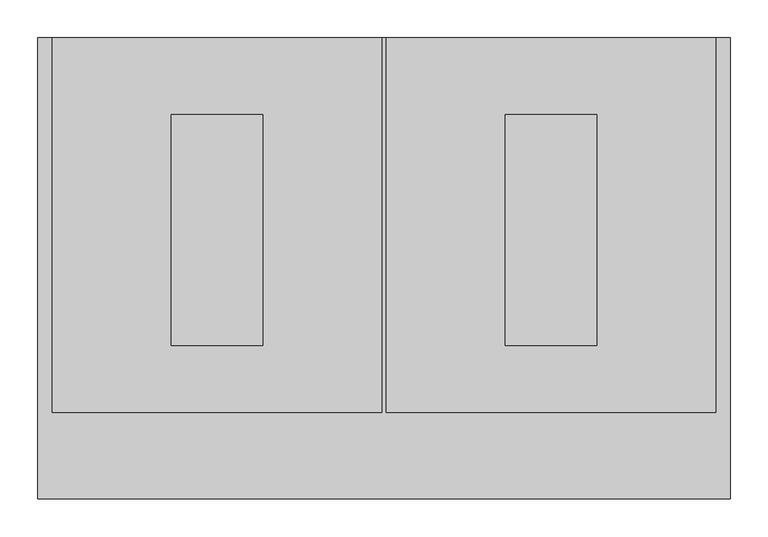
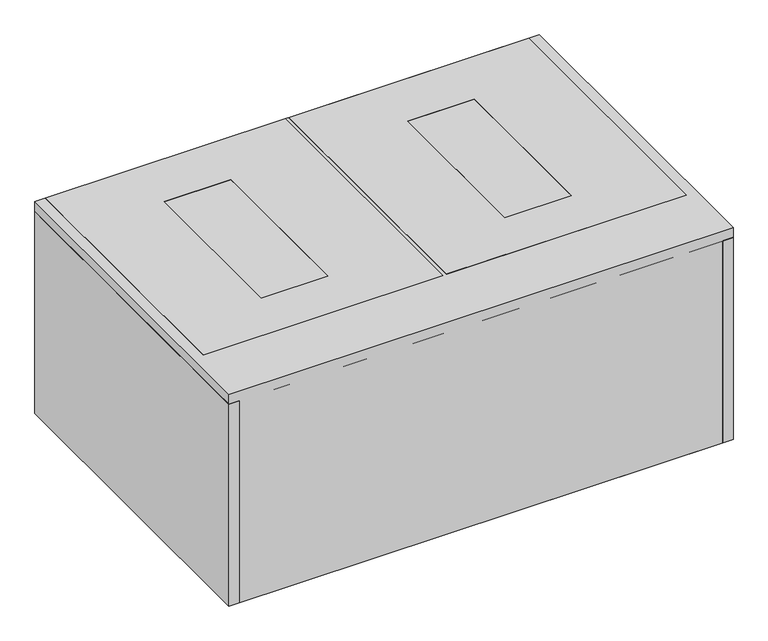
"""IFC4 building model written with IfcOpenShell, lengths in millimetres: proxy geometry, D0685 - Cabinet, Storage, Dental Operatory, Wall MNTD : D0685 - Cabinet, Storage, Dental Operatory, Wall MNTD."""

import ifcopenshell
import ifcopenshell.guid

model = None  # the IFC model being written
_history = None  # IfcOwnerHistory: only IFC2X3 demands one
_inside = {}  # id of a spatial element -> (the spatial element, [elements in it])
_under = {}  # id of a project, library or spatial element -> (it, [spatial elements below it])
_declared = {}  # id of a project -> (the project, [libraries it declares])
_typed = {}  # id of a type object -> (the type object, [elements of that type])
_made_of = {}  # id of a material, layer set ... -> (it, [elements and type objects made of it])


def new_model(schema):
    """Start an empty IFC model of exactly this schema.

    Asked for "IFC4X3", IfcOpenShell would pick the latest addendum, in which some entities
    have other attributes; the version numbers below select the first issue.
    IFC2X3 requires an IfcOwnerHistory on every rooted entity: one is made here for all.
    """
    global model, _history
    if schema == "IFC4X3":
        model = ifcopenshell.file(schema_version=(4, 3, 0, 0))
    else:
        model = ifcopenshell.file(schema=schema)
    _inside.clear()
    _under.clear()
    _declared.clear()
    _typed.clear()
    _made_of.clear()
    _history = None
    if model.schema == "IFC2X3":
        org = make("IfcOrganization", Name="unknown")
        user = make(
            "IfcPersonAndOrganization",
            ThePerson=make("IfcPerson", FamilyName="unknown"),
            TheOrganization=org,
        )
        app = make(
            "IfcApplication",
            ApplicationDeveloper=org,
            Version="unknown",
            ApplicationFullName="unknown",
            ApplicationIdentifier="unknown",
        )
        _history = make(
            "IfcOwnerHistory",
            OwningUser=user,
            OwningApplication=app,
            ChangeAction="ADDED",
            CreationDate=0,
        )
    return model


def make(cls, **values):
    """One entity of the class cls with the attributes given. An attribute that is None is left unset."""
    return model.create_entity(
        cls, **{name: value for name, value in values.items() if value is not None}
    )


def rooted(cls, **values):
    """An entity with a GlobalId (a new one), such as an element, a storey or a relation."""
    return make(cls, GlobalId=ifcopenshell.guid.new(), OwnerHistory=_history, **values)


def si_unit(unit_type, name, prefix=None):
    """IfcSIUnit, for example si_unit("LENGTHUNIT", "METRE", prefix="MILLI")."""
    return make("IfcSIUnit", UnitType=unit_type, Prefix=prefix, Name=name)


def assignment(units):
    """IfcUnitAssignment: the units of a project."""
    return None if units is None else make("IfcUnitAssignment", Units=units)


def point(xyz):
    """IfcCartesianPoint."""
    return None if xyz is None else make("IfcCartesianPoint", Coordinates=xyz)


def direction(xyz):
    """IfcDirection."""
    return None if xyz is None else make("IfcDirection", DirectionRatios=xyz)


def frame(location, z_axis=None, x_axis=None):
    """IfcAxis2Placement3D, a coordinate frame: its origin and axes. An axis left out is left unset."""
    return make(
        "IfcAxis2Placement3D",
        Location=point(location),
        Axis=direction(z_axis),
        RefDirection=direction(x_axis),
    )


def origin():
    """The frame at (0, 0, 0) with its axes left unset."""
    return frame((0.0, 0.0, 0.0))


def origin_with_axes():
    """The frame at (0, 0, 0) with the z axis (0, 0, 1) and the x axis (1, 0, 0) written out."""
    return frame((0.0, 0.0, 0.0), z_axis=(0.0, 0.0, 1.0), x_axis=(1.0, 0.0, 0.0))


def place(relative_to, where):
    """IfcLocalPlacement: puts the frame where relative to a parent placement (None: the world)."""
    return make(
        "IfcLocalPlacement", PlacementRelTo=relative_to, RelativePlacement=where
    )


def context(
    kind, dimensions, precision=None, world=None, true_north=None, identifier=None
):
    """IfcGeometricRepresentationContext, for example the 3D "Model" context."""
    return make(
        "IfcGeometricRepresentationContext",
        ContextIdentifier=identifier,
        ContextType=kind,
        CoordinateSpaceDimension=dimensions,
        Precision=precision,
        WorldCoordinateSystem=world,
        TrueNorth=true_north,
    )


def project(units=None, contexts=None):
    """IfcProject with its units and contexts."""
    return rooted(
        "IfcProject",
        Name="project",
        RepresentationContexts=contexts,
        UnitsInContext=assignment(units),
    )


def spatial(cls, under=None, at=None, **own):
    """A site, building, storey or space (cls), placed at a placement, below another one or the project."""
    s = rooted(cls, ObjectPlacement=at, **own)
    if under is not None:
        _under.setdefault(under.id(), (under, []))[1].append(s)
    return s


def polyline(points):
    """IfcPolyline through the points."""
    return make("IfcPolyline", Points=[point(p) for p in points])


def outline(outer, holes=None, kind="AREA"):
    """IfcArbitraryClosedProfileDef: a profile drawn as a closed curve; with holes, ...WithVoids."""
    if holes is None:
        return make("IfcArbitraryClosedProfileDef", ProfileType=kind, OuterCurve=outer)
    return make(
        "IfcArbitraryProfileDefWithVoids",
        ProfileType=kind,
        OuterCurve=outer,
        InnerCurves=holes,
    )


def extrude(swept, where, along, depth):
    """IfcExtrudedAreaSolid: the profile swept, set in the frame where, extruded along a direction by depth."""
    return make(
        "IfcExtrudedAreaSolid",
        SweptArea=swept,
        Position=where,
        ExtrudedDirection=direction(along),
        Depth=depth,
    )


def faces_of(points, faces, orient=None, outer=None):
    """IfcFace entities. A face is a list of loops; a loop is a list of indices into points, from 0.

    orient and outer hold one flag for each loop. By default every Orientation is true, the
    first loop of a face is its IfcFaceOuterBound and the others are IfcFaceBound.
    """
    made = []
    for i, loops in enumerate(faces):
        bounds = []
        for j, loop in enumerate(loops):
            is_outer = j == 0 if outer is None else outer[i][j]
            bounds.append(
                make(
                    "IfcFaceOuterBound" if is_outer else "IfcFaceBound",
                    Bound=make("IfcPolyLoop", Polygon=[points[k] for k in loop]),
                    Orientation=True if orient is None else orient[i][j],
                )
            )
        made.append(make("IfcFace", Bounds=bounds))
    return made


def faceted_brep(points, faces, orient=None, outer=None, voids=None):
    """IfcFacetedBrep: a solid bounded by flat faces; with voids (closed shells), ...WithVoids."""
    shared = [point(p) for p in points]
    hull = make("IfcClosedShell", CfsFaces=faces_of(shared, faces, orient, outer))
    if voids is None:
        return make("IfcFacetedBrep", Outer=hull)
    return make(
        "IfcFacetedBrepWithVoids",
        Outer=hull,
        Voids=[
            make(cls, CfsFaces=faces_of(shared, fs, o, b)) for cls, fs, o, b in voids
        ],
    )


def shape(context_of_items, identifier, shape_type, items):
    """IfcShapeRepresentation: the items that make up one representation, for example the "Body"."""
    return make(
        "IfcShapeRepresentation",
        ContextOfItems=context_of_items,
        RepresentationIdentifier=identifier,
        RepresentationType=shape_type,
        Items=items,
    )


def source(mapping_origin, context_of_items, identifier, shape_type, items):
    """IfcRepresentationMap: a shape defined once, which mapped items show again and again."""
    return make(
        "IfcRepresentationMap",
        MappingOrigin=mapping_origin,
        MappedRepresentation=shape(context_of_items, identifier, shape_type, items),
    )


def transform(
    local_origin,
    x_axis=None,
    y_axis=None,
    z_axis=None,
    scale=None,
    scale2=None,
    scale3=None,
    uniform=True,
):
    """IfcCartesianTransformationOperator3D, or its non-uniform kind. x_axis, y_axis, z_axis: its Axis1, 2, 3."""
    if uniform:
        return make(
            "IfcCartesianTransformationOperator3D",
            Axis1=direction(x_axis),
            Axis2=direction(y_axis),
            LocalOrigin=point(local_origin),
            Scale=scale,
            Axis3=direction(z_axis),
        )
    return make(
        "IfcCartesianTransformationOperator3DnonUniform",
        Axis1=direction(x_axis),
        Axis2=direction(y_axis),
        LocalOrigin=point(local_origin),
        Scale=scale,
        Axis3=direction(z_axis),
        Scale2=scale2,
        Scale3=scale3,
    )


def mapped(mapping_source, mapping_target):
    """IfcMappedItem: shows the shape of a source again, moved by a transform."""
    return make(
        "IfcMappedItem", MappingSource=mapping_source, MappingTarget=mapping_target
    )


def made_of(thing, what):
    """Note that an element or type object is made of a material, layer set ...; save() writes the relation."""
    if what is not None:
        _made_of.setdefault(what.id(), (what, []))[1].append(thing)
    return thing


def element(
    cls,
    number,
    at=None,
    inside=None,
    cuts=None,
    type_object=None,
    material=None,
    context=None,
    identifier="Body",
    shape_type=None,
    held_by="IfcProductDefinitionShape",
    body=None,
    shapes=None,
    **own,
):
    """One element of the class cls, such as IfcWall. Its Tag is "e" and its number.

    at: its placement. inside: the storey or other place that contains it. cuts: it is an
    opening in that element (IfcRelVoidsElement). A single representation is given by context,
    identifier, shape_type and body (its items); several are given by shapes. held_by: the class
    of the entity that holds the representations. save() writes the other relations.
    """
    e = rooted(cls, Tag="e%d" % number, ObjectPlacement=at, **own)
    if body is not None:
        shapes = [shape(context, identifier, shape_type, body)]
    if shapes is not None:
        e.Representation = make(held_by, Representations=shapes)
    if inside is not None:
        _inside.setdefault(inside.id(), (inside, []))[1].append(e)
    if cuts is not None:
        rooted(
            "IfcRelVoidsElement", RelatingBuildingElement=cuts, RelatedOpeningElement=e
        )
    if type_object is not None:
        _typed.setdefault(type_object.id(), (type_object, []))[1].append(e)
    return made_of(e, material)


def aggregate(whole, parts):
    """IfcRelAggregates: a whole, such as a stair, and the parts it consists of."""
    return rooted("IfcRelAggregates", RelatingObject=whole, RelatedObjects=parts)


def save(model, path):
    """Write the relations noted so far, then the file.

    IfcRelAggregates (storeys below a building ...), IfcRelContainedInSpatialStructure (elements
    in a storey), IfcRelDefinesByType, IfcRelAssociatesMaterial and IfcRelDeclares: one each for
    every whole, place, type object, material and project.
    """
    for whole, parts in _under.values():
        aggregate(whole, parts)
    for where, things in _inside.values():
        rooted(
            "IfcRelContainedInSpatialStructure",
            RelatedElements=things,
            RelatingStructure=where,
        )
    for kind, things in _typed.values():
        rooted("IfcRelDefinesByType", RelatedObjects=things, RelatingType=kind)
    for what, things in _made_of.values():
        rooted("IfcRelAssociatesMaterial", RelatedObjects=things, RelatingMaterial=what)
    for by, libraries in _declared.values():
        rooted("IfcRelDeclares", RelatingContext=by, RelatedDefinitions=libraries)
    model.write(path)


def specialty_equipment_dde70959(model_context):
    return source(origin(), model_context, "Body", "SolidModel", [
        faceted_brep([(438.15, 101.6, 387.35), (438.15, 609.6, 387.35), (438.15, 609.6, 406.4), (438.15, 114.3, 406.4), (438.15, 114.3, 396.875), (438.15, 101.6, 396.875), (3.175, 101.6, 387.35), (3.175, 101.6, 396.875), (3.175, 114.3, 396.875), (3.175, 114.3, 406.4), (3.175, 609.6, 406.4), (3.175, 609.6, 387.35), (160.3375, 508.0, 387.35), (160.3375, 203.2, 387.35), (280.9875, 203.2, 387.35), (280.9875, 508.0, 387.35), (160.3375, 203.2, 406.4), (160.3375, 508.0, 406.4), (280.9875, 508.0, 406.4), (280.9875, 203.2, 406.4)], [[[0, 1, 2, 3, 4, 5]], [[6, 7, 8, 9, 10, 11]], [[1, 0, 6, 11], [12, 13, 14, 15]], [[2, 1, 11, 10]], [[3, 2, 10, 9], [16, 17, 18, 19]], [[4, 3, 9, 8]], [[5, 4, 8, 7]], [[0, 5, 7, 6]], [[16, 13, 12, 17]], [[13, 16, 19, 14]], [[14, 19, 18, 15]], [[17, 12, 15, 18]]]),
        faceted_brep([(-3.175, 101.6, 387.35), (-3.175, 609.6, 387.35), (-3.175, 609.6, 406.4), (-3.175, 114.3, 406.4), (-3.175, 114.3, 396.875), (-3.175, 101.6, 396.875), (-438.15, 101.6, 387.35), (-438.15, 101.6, 396.875), (-438.15, 114.3, 396.875), (-438.15, 114.3, 406.4), (-438.15, 609.6, 406.4), (-438.15, 609.6, 387.35), (-160.3375, 508.0, 387.35), (-280.9875, 508.0, 387.35), (-280.9875, 203.2, 387.35), (-160.3375, 203.2, 387.35), (-280.9875, 508.0, 406.4), (-160.3375, 508.0, 406.4), (-160.3375, 203.2, 406.4), (-280.9875, 203.2, 406.4)], [[[0, 1, 2, 3, 4, 5]], [[6, 7, 8, 9, 10, 11]], [[1, 0, 6, 11], [12, 13, 14, 15]], [[2, 1, 11, 10]], [[3, 2, 10, 9], [16, 17, 18, 19]], [[4, 3, 9, 8]], [[5, 4, 8, 7]], [[0, 5, 7, 6]], [[16, 13, 12, 17]], [[13, 16, 19, 14]], [[14, 19, 18, 15]], [[17, 12, 15, 18]]]),
        extrude(outline(polyline([(-160.3375, 508.0), (-160.3375, 203.2), (-280.9875, 203.2), (-280.9875, 508.0), (-160.3375, 508.0)])), frame((0.0, 0.0, 396.875), z_axis=(0.0, 0.0, 1.0), x_axis=(1.0, 0.0, 0.0)), (0.0, 0.0, 1.0), 9.525),
        extrude(outline(polyline([(280.9875, 508.0), (280.9875, 203.2), (160.3375, 203.2), (160.3375, 508.0), (280.9875, 508.0)])), frame((0.0, 0.0, 396.875), z_axis=(0.0, 0.0, 1.0), x_axis=(1.0, 0.0, 0.0)), (0.0, 0.0, 1.0), 9.525),
        extrude(outline(polyline([(457.2, 0.0), (438.15, 0.0), (438.15, 609.6), (457.2, 609.6), (457.2, 0.0)])), origin_with_axes(), (0.0, 0.0, 1.0), 387.35),
        extrude(outline(polyline([(-438.15, 0.0), (-457.2, 0.0), (-457.2, 609.6), (-438.15, 609.6), (-438.15, 0.0)])), origin_with_axes(), (0.0, 0.0, 1.0), 387.35),
        extrude(outline(polyline([(457.2, 609.6), (457.2, 0.0), (-457.2, 0.0), (-457.2, 609.6), (457.2, 609.6)])), origin_with_axes(), (0.0, 0.0, 1.0), 406.4),
        extrude(outline(polyline([(438.15, 427.0375), (-438.15, 427.0375), (-438.15, 439.7375), (438.15, 439.7375), (438.15, 427.0375)])), frame((0.0, 0.0, 19.05), z_axis=(0.0, 0.0, 1.0), x_axis=(1.0, 0.0, 0.0)), (0.0, 0.0, 1.0), 368.3),
        extrude(outline(polyline([(438.15, 265.1125), (-438.15, 265.1125), (-438.15, 277.8125), (438.15, 277.8125), (438.15, 265.1125)])), frame((0.0, 0.0, 19.05), z_axis=(0.0, 0.0, 1.0), x_axis=(1.0, 0.0, 0.0)), (0.0, 0.0, 1.0), 368.3),
        extrude(outline(polyline([(-438.15, 609.6), (438.15, 609.6), (438.15, 590.55), (-438.15, 590.55), (-438.15, 609.6)])), origin_with_axes(), (0.0, 0.0, 1.0), 387.35),
        extrude(outline(polyline([(438.15, 609.6), (438.15, 101.6), (-438.15, 101.6), (-438.15, 609.6), (438.15, 609.6)])), origin_with_axes(), (0.0, 0.0, 1.0), 19.05),
        extrude(outline(polyline([(-438.15, 101.6), (438.15, 101.6), (438.15, 0.0), (-438.15, 0.0), (-438.15, 101.6)])), origin_with_axes(), (0.0, 0.0, 1.0), 387.35),
    ])


if __name__ == "__main__":
    model = new_model("IFC4")
    model_context = context("Model", 3, world=origin())
    ifc_project = project(units=[si_unit("LENGTHUNIT", "METRE", prefix="MILLI")], contexts=[model_context])
    site = spatial("IfcSite", under=ifc_project)
    building = spatial("IfcBuilding", under=site)
    placement = place(None, origin())
    specialty_equipment_shape = specialty_equipment_dde70959(model_context)
    element("IfcBuildingElementProxy", 1, Name="D0685 - Cabinet, Storage, Dental Operatory, Wall MNTD : D0685 - Cabinet, Storage, Dental Operatory, Wall MNTD", ObjectType="D0685 - Cabinet, Storage, Dental Operatory, Wall MNTD : D0685 - Cabinet, Storage, Dental Operatory, Wall MNTD", at=placement, inside=building, context=model_context, shape_type="MappedRepresentation", body=[
        mapped(specialty_equipment_shape, transform((0.0, 0.0, 0.0), x_axis=(1.0, 0.0, 0.0), y_axis=(0.0, 1.0, 0.0), z_axis=(0.0, 0.0, 1.0))),
    ])
    save(model, "model.ifc")

# Revit data of these elements
# Type "D0685 - Cabinet, Storage, Dental Operatory, Wall MNTD : D0685 - Cabinet, Storage, Dental Operatory, Wall MNTD"
#   Watts2 = "0"
#   Watts1 = "0"
#   Unit_Issue = "EA"
#   UTIL_6_Misc = "-"
#   UTIL_5_NonMedGas = "-"
#   UTIL_4_MiscGas = "-"
#   UTIL_3_MedGas = "-"
#   UTIL_2_Elec = "-"
#   UTIL_1_WaterDrain = "-"
#   Nomenclature = "Cabinet, Storage, Dental Operatory, Wall MNTD"
#   NSN = "6520"
#   Location [instance default] = ""
#   JSN = "D0685"
#   Fund_Source_VA = "-"
#   Fund_Source_Navy = "-"
#   Fund_Source_Army = "-"
#   Fund_Source_AF = "-"
#   ELEC_Volts2 = "0"
#   ELEC_Volts1 = "0"
#   ELEC_Phase2 = "0"
#   ELEC_Phase1 = "0"
#   ELEC_HertzSwitch = "0"
#   ELEC_HertzDependent = "0"
#   ELEC_Hertz = "0"
#   ELEC_Amps2 = "0"
#   ELEC_Amps1 = "0"
#   DetailDescription = "An upper wall mounted storage cabinet with two adjustable shelves providing additional space for dental supplies and equipment in a dental operative. Cabinet is approximately 34\"W x 12\"D x 24\"H with other widths available. Cabinet is frequently mounted above JSN D0680, Console, Accessory/Side, Dental Operatory."
#   CAT_VA = "A"
#   CAT_Navy = "A"
#   CAT_IHS = "-"
#   CAT_Army = "A"
#   CAT_AF = "A"
#   BTUperhour = "0"
#   Weight_IP = 0
#   Default Elevation = 4' - 6"
#   DIM_Width_IP = 3' - 0"
#   DIM_Height_IP = 2' - 0"
#   DIM_Depth_IP = 1' - 4"
#   Top Panel Material = none
#   Side Panel Material = none
#   Shelf Panel Material = none
#   Door Panel Material = none
#   Door Glass Material = none
#   Back Panel Material = none
#   Assembly Code = ""
# Element 1 (IfcBuildingElementProxy, "D0685 - Cabinet, Storage, Dental Operatory, Wall MNTD : D0685 - Cabinet, Storage, Dental Operatory, Wall MNTD")
#   Materials on its faces: "CabinetFinish", "Glass", "EquipSpace"
# Materials
#   "CabinetFinish": class "Unassigned", colour RGB 245 239 218, transparency 0
#   "Glass": class "Glass", colour RGB 0 128 192, transparency 0.75
#   "EquipSpace": class "Unassigned", colour RGB 221 217 195, transparency 0.5
